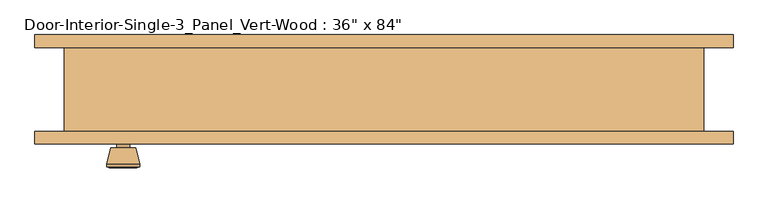
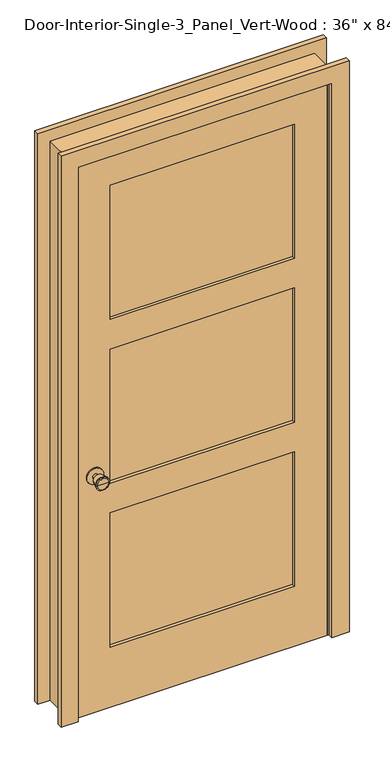
"""IFC4 building model written with IfcOpenShell, lengths in millimetres: door geometry."""

from ifc_helpers import new_model, si_unit, point, frame, frame_2d, origin, place, context, project, spatial, polyline, circle_curve, trimmed, segment, composite_curve, outline, extrude, faceted_brep, source, transform, mapped, element, save
from ifc_brep_helpers import plane_surface, cylinder_surface, revolved_surface, advanced_brep


def door_78a51fc2(model_context):
    return source(origin(), model_context, "Body", "SolidModel", [
        advanced_brep(
        [(-393.7, -19.4, 914.4), (-403.7, -19.4, 914.4), (-383.7, -19.4, 914.4), (-373.2241324, 29.6, 914.4), (-414.1758676, 29.6, 914.4), (-393.7, 29.6, 914.4), (-368.7, 27.7721319, 914.4), (-418.7, 27.7721319, 914.4), (-368.7, 24.3084537, 914.4), (-418.7, 24.3084537, 914.4), (-375.063764, -0.4, 914.4), (-412.336236, -0.4, 914.4), (-383.7, -0.4, 914.4), (-403.7, -0.4, 914.4)],
        [
            (0, 1),
            (1, 2, circle_curve(frame((-393.7, -19.4, 914.4), z_axis=(0.0, -1.0, 0.0), x_axis=(-1.0, 0.0, 0.0)), 10.0)),
            (2, 0),
            (2, 1, circle_curve(frame((-393.7, -19.4, 914.4), z_axis=(0.0, -1.0, 0.0), x_axis=(-1.0, 0.0, 0.0)), 10.0)),
            (3, 4, circle_curve(frame((-393.7, 29.6, 914.4), z_axis=(0.0, 1.0, 0.0), x_axis=(-1.0, 0.0, 0.0)), 20.4758676)),
            (4, 5),
            (5, 3),
            (4, 3, circle_curve(frame((-393.7, 29.6, 914.4), z_axis=(0.0, 1.0, 0.0), x_axis=(-1.0, 0.0, 0.0)), 20.4758676)),
            (6, 7, circle_curve(frame((-393.7, 27.7721319, 914.4), z_axis=(0.0, 1.0, 0.0), x_axis=(-1.0, 0.0, 0.0)), 25.0)),
            (7, 4),
            (3, 6),
            (7, 6, circle_curve(frame((-393.7, 27.7721319, 914.4), z_axis=(0.0, 1.0, 0.0), x_axis=(-1.0, 0.0, 0.0)), 25.0)),
            (8, 9, circle_curve(frame((-393.7, 24.3084537, 914.4), z_axis=(0.0, 1.0, 0.0), x_axis=(-1.0, 0.0, 0.0)), 25.0)),
            (9, 7),
            (6, 8),
            (9, 8, circle_curve(frame((-393.7, 24.3084537, 914.4), z_axis=(0.0, 1.0, 0.0), x_axis=(-1.0, 0.0, 0.0)), 25.0)),
            (10, 11, circle_curve(frame((-393.7, -0.4, 914.4), z_axis=(0.0, 1.0, 0.0), x_axis=(-1.0, 0.0, 0.0)), 18.636236)),
            (11, 9),
            (8, 10),
            (11, 10, circle_curve(frame((-393.7, -0.4, 914.4), z_axis=(0.0, 1.0, 0.0), x_axis=(-1.0, 0.0, 0.0)), 18.636236)),
            (12, 13, circle_curve(frame((-393.7, -0.4, 914.4), z_axis=(0.0, 1.0, 0.0), x_axis=(-1.0, 0.0, 0.0)), 10.0)),
            (13, 11),
            (10, 12),
            (13, 12, circle_curve(frame((-393.7, -0.4, 914.4), z_axis=(0.0, 1.0, 0.0), x_axis=(-1.0, 0.0, 0.0)), 10.0)),
            (1, 13),
            (12, 2),
        ],
        [
            plane_surface(frame((-393.7, -19.4, 914.4), z_axis=(0.0, -1.0, 0.0), x_axis=(-1.0, 0.0, 0.0))),
            plane_surface(frame((-393.7, 29.6, 914.4), z_axis=(0.0, 1.0, 0.0), x_axis=(-1.0, 0.0, 0.0))),
            revolved_surface(polyline([(-414.1758676, 29.6, 914.4), (-418.7, 27.7721319, 914.4)]), (-393.7, -19.4, 914.4), (0.0, -1.0, 0.0)),
            cylinder_surface(frame((-393.7, -19.4, 914.4), z_axis=(0.0, -1.0, 0.0), x_axis=(-1.0, 0.0, 0.0)), 25.0),
            revolved_surface(polyline([(-418.7, 24.3084537, 914.4), (-412.336236, -0.4, 914.4)]), (-393.7, -19.4, 914.4), (0.0, -1.0, 0.0)),
            plane_surface(frame((-393.7, -0.4, 914.4), z_axis=(0.0, -1.0, 0.0), x_axis=(-1.0, 0.0, 0.0))),
            cylinder_surface(frame((-393.7, -19.4, 914.4), z_axis=(0.0, -1.0, 0.0), x_axis=(-1.0, 0.0, 0.0)), 10.0),
        ],
        [
            (0, [[1, 2, 3]]),
            (0, [[-3, 4, -1]]),
            (1, [[5, 6, 7]]),
            (1, [[8, -7, -6]]),
            (2, [[9, 10, -5, 11]]),
            (2, [[12, -11, -8, -10]]),
            (3, [[13, 14, -9, 15]]),
            (3, [[16, -15, -12, -14]]),
            (4, [[17, 18, -13, 19]]),
            (4, [[20, -19, -16, -18]]),
            (5, [[21, 22, -17, 23]]),
            (5, [[24, -23, -20, -22]]),
            (6, [[-2, 25, -21, 26]]),
            (6, [[-4, -26, -24, -25]]),
        ],
    ),
        extrude(outline(composite_curve([segment(trimmed(circle_curve(frame_2d((914.4, -393.7)), 30.0), [point((914.4, -423.7))], [point((914.4, -363.7))], False, "CARTESIAN"), True, "CONTINUOUS"), segment(trimmed(circle_curve(frame_2d((914.4, -393.7)), 30.0), [point((914.4, -363.7))], [point((914.4, -423.7))], False, "CARTESIAN"), True, "CONTINUOUS")], self_intersect=False)), frame((0.0, -25.4, 0.0), z_axis=(0.0, 1.0, 0.0), x_axis=(0.0, 0.0, 1.0)), (0.0, 0.0, 1.0), 6.0),
        advanced_brep(
        [(-393.7, -66.325, 914.4), (-383.7, -66.325, 914.4), (-403.7, -66.325, 914.4), (-373.2241324, -115.325, 914.4), (-393.7, -115.325, 914.4), (-414.1758676, -115.325, 914.4), (-368.7, -113.4971319, 914.4), (-418.7, -113.4971319, 914.4), (-368.7, -110.0334537, 914.4), (-418.7, -110.0334537, 914.4), (-375.063764, -85.325, 914.4), (-412.336236, -85.325, 914.4), (-383.7, -85.325, 914.4), (-403.7, -85.325, 914.4)],
        [
            (0, 1),
            (1, 2, circle_curve(frame((-393.7, -66.325, 914.4), z_axis=(0.0, 1.0, 0.0), x_axis=(-1.0, 0.0, 0.0)), 10.0)),
            (2, 0),
            (2, 1, circle_curve(frame((-393.7, -66.325, 914.4), z_axis=(0.0, 1.0, 0.0), x_axis=(-1.0, 0.0, 0.0)), 10.0)),
            (3, 4),
            (4, 5),
            (5, 3, circle_curve(frame((-393.7, -115.325, 914.4), z_axis=(0.0, -1.0, 0.0), x_axis=(-1.0, 0.0, 0.0)), 20.4758676)),
            (3, 5, circle_curve(frame((-393.7, -115.325, 914.4), z_axis=(0.0, -1.0, 0.0), x_axis=(-1.0, 0.0, 0.0)), 20.4758676)),
            (6, 3),
            (5, 7),
            (7, 6, circle_curve(frame((-393.7, -113.4971319, 914.4), z_axis=(0.0, -1.0, 0.0), x_axis=(-1.0, 0.0, 0.0)), 25.0)),
            (6, 7, circle_curve(frame((-393.7, -113.4971319, 914.4), z_axis=(0.0, -1.0, 0.0), x_axis=(-1.0, 0.0, 0.0)), 25.0)),
            (8, 6),
            (7, 9),
            (9, 8, circle_curve(frame((-393.7, -110.0334537, 914.4), z_axis=(0.0, -1.0, 0.0), x_axis=(-1.0, 0.0, 0.0)), 25.0)),
            (8, 9, circle_curve(frame((-393.7, -110.0334537, 914.4), z_axis=(0.0, -1.0, 0.0), x_axis=(-1.0, 0.0, 0.0)), 25.0)),
            (10, 8),
            (9, 11),
            (11, 10, circle_curve(frame((-393.7, -85.325, 914.4), z_axis=(0.0, -1.0, 0.0), x_axis=(-1.0, 0.0, 0.0)), 18.636236)),
            (10, 11, circle_curve(frame((-393.7, -85.325, 914.4), z_axis=(0.0, -1.0, 0.0), x_axis=(-1.0, 0.0, 0.0)), 18.636236)),
            (12, 10),
            (11, 13),
            (13, 12, circle_curve(frame((-393.7, -85.325, 914.4), z_axis=(0.0, -1.0, 0.0), x_axis=(-1.0, 0.0, 0.0)), 10.0)),
            (12, 13, circle_curve(frame((-393.7, -85.325, 914.4), z_axis=(0.0, -1.0, 0.0), x_axis=(-1.0, 0.0, 0.0)), 10.0)),
            (1, 12),
            (13, 2),
        ],
        [
            plane_surface(frame((-393.7, -66.325, 914.4), z_axis=(0.0, 1.0, 0.0), x_axis=(-1.0, 0.0, 0.0))),
            plane_surface(frame((-393.7, -115.325, 914.4), z_axis=(0.0, -1.0, 0.0), x_axis=(-1.0, 0.0, 0.0))),
            revolved_surface(polyline([(-414.1758676, -115.325, 914.4), (-418.7, -113.4971319, 914.4)]), (-393.7, -66.325, 914.4), (0.0, 1.0, 0.0)),
            cylinder_surface(frame((-393.7, -66.325, 914.4), z_axis=(0.0, 1.0, 0.0), x_axis=(-1.0, 0.0, 0.0)), 25.0),
            revolved_surface(polyline([(-418.7, -110.0334537, 914.4), (-412.336236, -85.325, 914.4)]), (-393.7, -66.325, 914.4), (0.0, 1.0, 0.0)),
            plane_surface(frame((-393.7, -85.325, 914.4), z_axis=(0.0, 1.0, 0.0), x_axis=(-1.0, 0.0, 0.0))),
            cylinder_surface(frame((-393.7, -66.325, 914.4), z_axis=(0.0, 1.0, 0.0), x_axis=(-1.0, 0.0, 0.0)), 10.0),
        ],
        [
            (0, [[1, 2, 3]]),
            (0, [[-3, 4, -1]]),
            (1, [[5, 6, 7]]),
            (1, [[-6, -5, 8]]),
            (2, [[9, -7, 10, 11]]),
            (2, [[-10, -8, -9, 12]]),
            (3, [[13, -11, 14, 15]]),
            (3, [[-14, -12, -13, 16]]),
            (4, [[17, -15, 18, 19]]),
            (4, [[-18, -16, -17, 20]]),
            (5, [[21, -19, 22, 23]]),
            (5, [[-22, -20, -21, 24]]),
            (6, [[25, -23, 26, -2]]),
            (6, [[-26, -24, -25, -4]]),
        ],
    ),
        extrude(outline(composite_curve([segment(trimmed(circle_curve(frame_2d((914.4, -393.7)), 30.0), [point((914.4, -423.7))], [point((914.4, -363.7))], False, "CARTESIAN"), True, "CONTINUOUS"), segment(trimmed(circle_curve(frame_2d((914.4, -393.7)), 30.0), [point((914.4, -363.7))], [point((914.4, -423.7))], False, "CARTESIAN"), True, "CONTINUOUS")], self_intersect=False)), frame((0.0, -66.325, 0.0), z_axis=(0.0, 1.0, 0.0), x_axis=(0.0, 0.0, 1.0)), (0.0, 0.0, 1.0), 6.0),
        extrude(outline(polyline([(336.55, -37.0416667), (336.55, -48.6833333), (-336.55, -48.6833333), (-336.55, -37.0416667), (336.55, -37.0416667)])), frame((0.0, 0.0, 1496.4833333), z_axis=(0.0, 0.0, 1.0), x_axis=(1.0, 0.0, 0.0)), (0.0, 0.0, 1.0), 518.0541667),
        extrude(outline(polyline([(336.55, -37.0416667), (336.55, -48.6833333), (-336.55, -48.6833333), (-336.55, -37.0416667), (336.55, -37.0416667)])), frame((0.0, 0.0, 231.775), z_axis=(0.0, 0.0, 1.0), x_axis=(1.0, 0.0, 0.0)), (0.0, 0.0, 1.0), 518.0541667),
        extrude(outline(polyline([(336.55, -37.0416667), (336.55, -48.6833333), (-336.55, -48.6833333), (-336.55, -37.0416667), (336.55, -37.0416667)])), frame((0.0, 0.0, 864.1291667), z_axis=(0.0, 0.0, 1.0), x_axis=(1.0, 0.0, 0.0)), (0.0, 0.0, 1.0), 518.0541667),
        extrude(outline(polyline([(2133.6, -457.2), (0.0, -457.2), (0.0, 457.2), (2133.6, 457.2), (2133.6, -457.2)]), holes=[polyline([(2014.5375, -336.55), (2014.5375, 336.55), (1496.4833333, 336.55), (1496.4833333, -336.55), (2014.5375, -336.55)]), polyline([(749.8291667, -336.55), (749.8291667, 336.55), (231.775, 336.55), (231.775, -336.55), (749.8291667, -336.55)]), polyline([(1382.1833333, -336.55), (1382.1833333, 336.55), (864.1291667, 336.55), (864.1291667, -336.55), (1382.1833333, -336.55)])]), frame((0.0, -60.325, 0.0), z_axis=(0.0, 1.0, 0.0), x_axis=(0.0, 0.0, 1.0)), (0.0, 0.0, 1.0), 34.925),
        faceted_brep([(482.6, -60.325, 0.0), (457.2, -60.325, 0.0), (457.2, -25.4, 0.0), (444.5, -25.4, 0.0), (444.5, 9.525, 0.0), (457.2, 9.525, 0.0), (457.2, 66.675, 0.0), (482.6, 66.675, 0.0), (482.6, 66.675, 2159.0), (482.6, -60.325, 2159.0), (457.2, 66.675, 2133.6), (-457.2, 66.675, 2133.6), (-457.2, 66.675, 0.0), (-482.6, 66.675, 0.0), (-482.6, 66.675, 2159.0), (457.2, 9.525, 2133.6), (444.5, 9.525, 2120.9), (-444.5, 9.525, 2120.9), (-444.5, 9.525, 0.0), (-457.2, 9.525, 0.0), (-457.2, 9.525, 2133.6), (444.5, -25.4, 2120.9), (457.2, -25.4, 2133.6), (-457.2, -25.4, 2133.6), (-457.2, -25.4, 0.0), (-444.5, -25.4, 0.0), (-444.5, -25.4, 2120.9), (457.2, -60.325, 2133.6), (-482.6, -60.325, 2159.0), (-482.6, -60.325, 0.0), (-457.2, -60.325, 0.0), (-457.2, -60.325, 2133.6)], [[[0, 1, 2, 3, 4, 5, 6, 7]], [[7, 8, 9, 0]], [[6, 10, 11, 12, 13, 14, 8, 7]], [[5, 15, 10, 6]], [[4, 16, 17, 18, 19, 20, 15, 5]], [[3, 21, 16, 4]], [[2, 22, 23, 24, 25, 26, 21, 3]], [[1, 27, 22, 2]], [[0, 9, 28, 29, 30, 31, 27, 1]], [[8, 14, 28, 9]], [[15, 20, 11, 10]], [[21, 26, 17, 16]], [[27, 31, 23, 22]], [[29, 13, 12, 19, 18, 25, 24, 30]], [[14, 13, 29, 28]], [[20, 19, 12, 11]], [[26, 25, 18, 17]], [[31, 30, 24, 23]]]),
        extrude(outline(polyline([(0.0, 527.05), (2203.45, 527.05), (2203.45, -527.05), (0.0, -527.05), (0.0, -463.55), (2139.95, -463.55), (2139.95, 463.55), (0.0, 463.55), (0.0, 527.05)])), frame((0.0, 66.675, 0.0), z_axis=(0.0, 1.0, 0.0), x_axis=(0.0, 0.0, 1.0)), (0.0, 0.0, 1.0), 19.05),
        extrude(outline(polyline([(0.0, 527.05), (2203.45, 527.05), (2203.45, -527.05), (0.0, -527.05), (0.0, -463.55), (2139.95, -463.55), (2139.95, 463.55), (0.0, 463.55), (0.0, 527.05)])), frame((0.0, -79.375, 0.0), z_axis=(0.0, 1.0, 0.0), x_axis=(0.0, 0.0, 1.0)), (0.0, 0.0, 1.0), 19.05),
    ])


if __name__ == "__main__":
    model = new_model("IFC4")
    model_context = context("Model", 3, world=origin())
    ifc_project = project(units=[si_unit("LENGTHUNIT", "METRE", prefix="MILLI")], contexts=[model_context])
    site = spatial("IfcSite", under=ifc_project)
    building = spatial("IfcBuilding", under=site)
    placement = place(None, origin())
    door_shape = door_78a51fc2(model_context)
    element("IfcDoor", 1, ObjectType="Door-Interior-Single-3_Panel_Vert-Wood : 36\" x 84\"", at=placement, inside=building, context=model_context, shape_type="MappedRepresentation", body=[
        mapped(door_shape, transform((0.0, 0.0, 0.0), x_axis=(1.0, 0.0, 0.0), y_axis=(0.0, 1.0, 0.0), z_axis=(0.0, 0.0, 1.0))),
    ])
    save(model, "model.ifc")

# Revit data of these elements
# Type "Door-Interior-Single-3_Panel_Vert-Wood : 36\" x 84\""
#   Type Mark = "10"
#   Assembly Code = "C1020300"
#   Analytic Construction = "Wooden"
#   Top Rail = 0' - 4 11/16"
#   Thickness = 0' - 1 3/8"
#   Thermal Resistance (R) = 2.5876 (h·ft²·°F)/BTU
#   Swing Angle [instance default] = 90.00°
#   Stiles = 0' - 4 3/4"
#   Rough Width = 3' - 2"
#   Rough Height = 7' - 1"
#   Intermediate Rail = 0' - 4 1/2"
#   Height = 7' - 0"
#   Width = 3' - 0"
#   Heat Transfer Coefficient (U) = 0.3865 BTU/(h·ft²·°F)
#   Bottom Rail = 0' - 9 1/8"
#   Trim Material = Cherry
#   Panel Material = Cherry
#   Frame Material = Cherry
#   Door Handle Material = Aluminum
#   Visual Light Transmittance = 0
#   Solar Heat Gain Coefficient = 0
#   Wall Closure = (empty or 0)
#   Function = (empty or 0)
# Element 1 (IfcDoor, "Door-Interior-Single-3_Panel_Vert-Wood : 36\" x 84\"")
#   Materials on its faces: "Cherry", "Aluminum"
# Materials
#   "Cherry": class "Wood", colour RGB 226 177 128, transparency 0, Description = "Prunus Serotina", Cost = 0
#   "Aluminum": class "Metal", colour RGB 247 247 247, transparency 0, Description = "Aluminum 6061", Cost = 0
